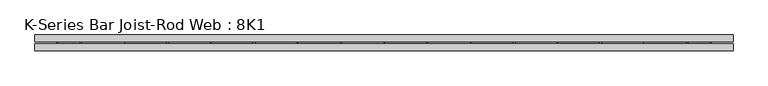
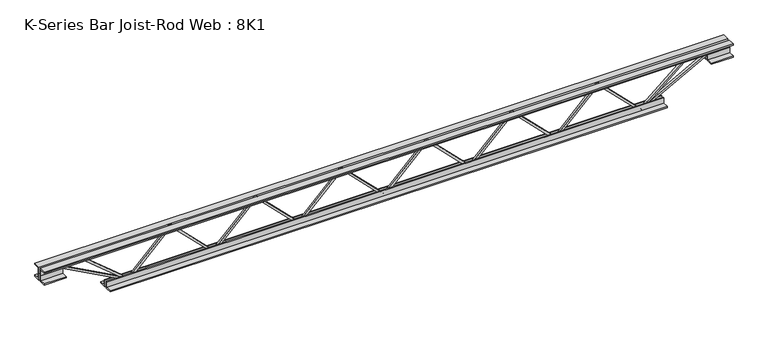
"""IFC4 building model written with IfcOpenShell, lengths in millimetres: beam geometry, K-Series Bar Joist-Rod Web : 8K1."""

import ifcopenshell
import ifcopenshell.guid

model = None  # the IFC model being written
_history = None  # IfcOwnerHistory: only IFC2X3 demands one
_inside = {}  # id of a spatial element -> (the spatial element, [elements in it])
_under = {}  # id of a project, library or spatial element -> (it, [spatial elements below it])
_declared = {}  # id of a project -> (the project, [libraries it declares])
_typed = {}  # id of a type object -> (the type object, [elements of that type])
_made_of = {}  # id of a material, layer set ... -> (it, [elements and type objects made of it])


def new_model(schema):
    """Start an empty IFC model of exactly this schema.

    Asked for "IFC4X3", IfcOpenShell would pick the latest addendum, in which some entities
    have other attributes; the version numbers below select the first issue.
    IFC2X3 requires an IfcOwnerHistory on every rooted entity: one is made here for all.
    """
    global model, _history
    if schema == "IFC4X3":
        model = ifcopenshell.file(schema_version=(4, 3, 0, 0))
    else:
        model = ifcopenshell.file(schema=schema)
    _inside.clear()
    _under.clear()
    _declared.clear()
    _typed.clear()
    _made_of.clear()
    _history = None
    if model.schema == "IFC2X3":
        org = make("IfcOrganization", Name="unknown")
        user = make(
            "IfcPersonAndOrganization",
            ThePerson=make("IfcPerson", FamilyName="unknown"),
            TheOrganization=org,
        )
        app = make(
            "IfcApplication",
            ApplicationDeveloper=org,
            Version="unknown",
            ApplicationFullName="unknown",
            ApplicationIdentifier="unknown",
        )
        _history = make(
            "IfcOwnerHistory",
            OwningUser=user,
            OwningApplication=app,
            ChangeAction="ADDED",
            CreationDate=0,
        )
    return model


def make(cls, **values):
    """One entity of the class cls with the attributes given. An attribute that is None is left unset."""
    return model.create_entity(
        cls, **{name: value for name, value in values.items() if value is not None}
    )


def rooted(cls, **values):
    """An entity with a GlobalId (a new one), such as an element, a storey or a relation."""
    return make(cls, GlobalId=ifcopenshell.guid.new(), OwnerHistory=_history, **values)


def si_unit(unit_type, name, prefix=None):
    """IfcSIUnit, for example si_unit("LENGTHUNIT", "METRE", prefix="MILLI")."""
    return make("IfcSIUnit", UnitType=unit_type, Prefix=prefix, Name=name)


def assignment(units):
    """IfcUnitAssignment: the units of a project."""
    return None if units is None else make("IfcUnitAssignment", Units=units)


def point(xyz):
    """IfcCartesianPoint."""
    return None if xyz is None else make("IfcCartesianPoint", Coordinates=xyz)


def direction(xyz):
    """IfcDirection."""
    return None if xyz is None else make("IfcDirection", DirectionRatios=xyz)


def frame(location, z_axis=None, x_axis=None):
    """IfcAxis2Placement3D, a coordinate frame: its origin and axes. An axis left out is left unset."""
    return make(
        "IfcAxis2Placement3D",
        Location=point(location),
        Axis=direction(z_axis),
        RefDirection=direction(x_axis),
    )


def origin():
    """The frame at (0, 0, 0) with its axes left unset."""
    return frame((0.0, 0.0, 0.0))


def place(relative_to, where):
    """IfcLocalPlacement: puts the frame where relative to a parent placement (None: the world)."""
    return make(
        "IfcLocalPlacement", PlacementRelTo=relative_to, RelativePlacement=where
    )


def context(
    kind, dimensions, precision=None, world=None, true_north=None, identifier=None
):
    """IfcGeometricRepresentationContext, for example the 3D "Model" context."""
    return make(
        "IfcGeometricRepresentationContext",
        ContextIdentifier=identifier,
        ContextType=kind,
        CoordinateSpaceDimension=dimensions,
        Precision=precision,
        WorldCoordinateSystem=world,
        TrueNorth=true_north,
    )


def project(units=None, contexts=None):
    """IfcProject with its units and contexts."""
    return rooted(
        "IfcProject",
        Name="project",
        RepresentationContexts=contexts,
        UnitsInContext=assignment(units),
    )


def spatial(cls, under=None, at=None, **own):
    """A site, building, storey or space (cls), placed at a placement, below another one or the project."""
    s = rooted(cls, ObjectPlacement=at, **own)
    if under is not None:
        _under.setdefault(under.id(), (under, []))[1].append(s)
    return s


def polyline(points):
    """IfcPolyline through the points."""
    return make("IfcPolyline", Points=[point(p) for p in points])


def outline(outer, holes=None, kind="AREA"):
    """IfcArbitraryClosedProfileDef: a profile drawn as a closed curve; with holes, ...WithVoids."""
    if holes is None:
        return make("IfcArbitraryClosedProfileDef", ProfileType=kind, OuterCurve=outer)
    return make(
        "IfcArbitraryProfileDefWithVoids",
        ProfileType=kind,
        OuterCurve=outer,
        InnerCurves=holes,
    )


def extrude(swept, where, along, depth):
    """IfcExtrudedAreaSolid: the profile swept, set in the frame where, extruded along a direction by depth."""
    return make(
        "IfcExtrudedAreaSolid",
        SweptArea=swept,
        Position=where,
        ExtrudedDirection=direction(along),
        Depth=depth,
    )


def shape(context_of_items, identifier, shape_type, items):
    """IfcShapeRepresentation: the items that make up one representation, for example the "Body"."""
    return make(
        "IfcShapeRepresentation",
        ContextOfItems=context_of_items,
        RepresentationIdentifier=identifier,
        RepresentationType=shape_type,
        Items=items,
    )


def source(mapping_origin, context_of_items, identifier, shape_type, items):
    """IfcRepresentationMap: a shape defined once, which mapped items show again and again."""
    return make(
        "IfcRepresentationMap",
        MappingOrigin=mapping_origin,
        MappedRepresentation=shape(context_of_items, identifier, shape_type, items),
    )


def transform(
    local_origin,
    x_axis=None,
    y_axis=None,
    z_axis=None,
    scale=None,
    scale2=None,
    scale3=None,
    uniform=True,
):
    """IfcCartesianTransformationOperator3D, or its non-uniform kind. x_axis, y_axis, z_axis: its Axis1, 2, 3."""
    if uniform:
        return make(
            "IfcCartesianTransformationOperator3D",
            Axis1=direction(x_axis),
            Axis2=direction(y_axis),
            LocalOrigin=point(local_origin),
            Scale=scale,
            Axis3=direction(z_axis),
        )
    return make(
        "IfcCartesianTransformationOperator3DnonUniform",
        Axis1=direction(x_axis),
        Axis2=direction(y_axis),
        LocalOrigin=point(local_origin),
        Scale=scale,
        Axis3=direction(z_axis),
        Scale2=scale2,
        Scale3=scale3,
    )


def mapped(mapping_source, mapping_target):
    """IfcMappedItem: shows the shape of a source again, moved by a transform."""
    return make(
        "IfcMappedItem", MappingSource=mapping_source, MappingTarget=mapping_target
    )


def made_of(thing, what):
    """Note that an element or type object is made of a material, layer set ...; save() writes the relation."""
    if what is not None:
        _made_of.setdefault(what.id(), (what, []))[1].append(thing)
    return thing


def element(
    cls,
    number,
    at=None,
    inside=None,
    cuts=None,
    type_object=None,
    material=None,
    context=None,
    identifier="Body",
    shape_type=None,
    held_by="IfcProductDefinitionShape",
    body=None,
    shapes=None,
    **own,
):
    """One element of the class cls, such as IfcWall. Its Tag is "e" and its number.

    at: its placement. inside: the storey or other place that contains it. cuts: it is an
    opening in that element (IfcRelVoidsElement). A single representation is given by context,
    identifier, shape_type and body (its items); several are given by shapes. held_by: the class
    of the entity that holds the representations. save() writes the other relations.
    """
    e = rooted(cls, Tag="e%d" % number, ObjectPlacement=at, **own)
    if body is not None:
        shapes = [shape(context, identifier, shape_type, body)]
    if shapes is not None:
        e.Representation = make(held_by, Representations=shapes)
    if inside is not None:
        _inside.setdefault(inside.id(), (inside, []))[1].append(e)
    if cuts is not None:
        rooted(
            "IfcRelVoidsElement", RelatingBuildingElement=cuts, RelatedOpeningElement=e
        )
    if type_object is not None:
        _typed.setdefault(type_object.id(), (type_object, []))[1].append(e)
    return made_of(e, material)


def aggregate(whole, parts):
    """IfcRelAggregates: a whole, such as a stair, and the parts it consists of."""
    return rooted("IfcRelAggregates", RelatingObject=whole, RelatedObjects=parts)


def save(model, path):
    """Write the relations noted so far, then the file.

    IfcRelAggregates (storeys below a building ...), IfcRelContainedInSpatialStructure (elements
    in a storey), IfcRelDefinesByType, IfcRelAssociatesMaterial and IfcRelDeclares: one each for
    every whole, place, type object, material and project.
    """
    for whole, parts in _under.values():
        aggregate(whole, parts)
    for where, things in _inside.values():
        rooted(
            "IfcRelContainedInSpatialStructure",
            RelatedElements=things,
            RelatingStructure=where,
        )
    for kind, things in _typed.values():
        rooted("IfcRelDefinesByType", RelatedObjects=things, RelatingType=kind)
    for what, things in _made_of.values():
        rooted("IfcRelAssociatesMaterial", RelatedObjects=things, RelatingMaterial=what)
    for by, libraries in _declared.values():
        rooted("IfcRelDeclares", RelatingContext=by, RelatedDefinitions=libraries)
    model.write(path)


def k_series_bar_joist_rod_web_8k1_291a3e72(model_context):
    return source(origin(), model_context, "Body", "SweptSolid", [
        extrude(outline(polyline([(-90.4875, 394.3021306), (-100.0125, 394.3021306), (-100.0125, 399.4476203), (90.4875, 590.2486857), (90.4875, 592.6577063), (-100.0125, 783.4587716), (-100.0125, 788.6042613), (-90.4875, 788.6042613), (-90.4875, 787.399751), (100.0125, 596.5986857), (100.0125, 586.3077063), (-90.4875, 395.506641), (-90.4875, 394.3021306)])), frame((0.0, -4.7625, 0.0), z_axis=(0.0, 1.0, 0.0), x_axis=(0.0, 0.0, 1.0)), (0.0, 0.0, 1.0), 9.525),
        extrude(outline(polyline([(-90.4875, 0.0), (-100.0125, 0.0), (-100.0125, 5.1454897), (90.4875, 195.946555), (90.4875, 198.3555756), (-100.0125, 389.156641), (-100.0125, 394.3021306), (-90.4875, 394.3021306), (-90.4875, 393.0976203), (100.0125, 202.296555), (100.0125, 192.0055756), (-90.4875, 1.2045103), (-90.4875, 0.0)])), frame((0.0, -4.7625, 0.0), z_axis=(0.0, 1.0, 0.0), x_axis=(0.0, 0.0, 1.0)), (0.0, 0.0, 1.0), 9.525),
        extrude(outline(polyline([(-90.4875, -394.3021306), (-100.0125, -394.3021306), (-100.0125, -389.156641), (90.4875, -198.3555756), (90.4875, -195.946555), (-100.0125, -5.1454897), (-100.0125, 0.0), (-90.4875, 0.0), (-90.4875, -1.2045103), (100.0125, -192.0055756), (100.0125, -202.296555), (-90.4875, -393.0976203), (-90.4875, -394.3021306)])), frame((0.0, -4.7625, 0.0), z_axis=(0.0, 1.0, 0.0), x_axis=(0.0, 0.0, 1.0)), (0.0, 0.0, 1.0), 9.525),
        extrude(outline(polyline([(-90.4875, -788.6042613), (-100.0125, -788.6042613), (-100.0125, -783.4587716), (90.4875, -592.6577063), (90.4875, -590.2486857), (-100.0125, -399.4476203), (-100.0125, -394.3021306), (-90.4875, -394.3021306), (-90.4875, -395.506641), (100.0125, -586.3077063), (100.0125, -596.5986857), (-90.4875, -787.399751), (-90.4875, -788.6042613)])), frame((0.0, -4.7625, 0.0), z_axis=(0.0, 1.0, 0.0), x_axis=(0.0, 0.0, 1.0)), (0.0, 0.0, 1.0), 9.525),
        extrude(outline(polyline([(-90.4875, 788.6042613), (-100.0125, 788.6042613), (-100.0125, 793.749751), (90.4875, 984.5508163), (90.4875, 986.9598369), (-100.0125, 1177.7609023), (-100.0125, 1182.9063919), (-90.4875, 1182.9063919), (-90.4875, 1181.7018816), (100.0125, 990.9008163), (100.0125, 980.6098369), (-90.4875, 789.8087716), (-90.4875, 788.6042613)])), frame((0.0, -4.7625, 0.0), z_axis=(0.0, 1.0, 0.0), x_axis=(0.0, 0.0, 1.0)), (0.0, 0.0, 1.0), 9.525),
        extrude(outline(polyline([(-90.4875, -1182.9063919), (-100.0125, -1182.9063919), (-100.0125, -1177.7609023), (90.4875, -986.9598369), (90.4875, -984.5508163), (-100.0125, -793.749751), (-100.0125, -788.6042613), (-90.4875, -788.6042613), (-90.4875, -789.8087716), (100.0125, -980.6098369), (100.0125, -990.9008163), (-90.4875, -1181.7018816), (-90.4875, -1182.9063919)])), frame((0.0, -4.7625, 0.0), z_axis=(0.0, 1.0, 0.0), x_axis=(0.0, 0.0, 1.0)), (0.0, 0.0, 1.0), 9.525),
        extrude(outline(polyline([(4.7625, 101.6), (36.5125, 101.6), (36.5125, 95.25), (11.1125, 95.25), (11.1125, 69.85), (4.7625, 69.85), (4.7625, 101.6)])), frame((-1589.3063919, 0.0, 0.0), z_axis=(1.0, 0.0, 0.0), x_axis=(0.0, 1.0, 0.0)), (0.0, 0.0, 1.0), 3178.6127839),
        extrude(outline(polyline([(-4.7625, 101.6), (-4.7625, 69.85), (-11.1125, 69.85), (-11.1125, 95.25), (-36.5125, 95.25), (-36.5125, 101.6), (-4.7625, 101.6)])), frame((-1589.3063919, 0.0, 0.0), z_axis=(1.0, 0.0, 0.0), x_axis=(0.0, 1.0, 0.0)), (0.0, 0.0, 1.0), 3178.6127839),
        extrude(outline(polyline([(-4.7625, 38.1), (-36.5125, 38.1), (-36.5125, 44.45), (-11.1125, 44.45), (-11.1125, 69.85), (-4.7625, 69.85), (-4.7625, 38.1)])), frame((-1589.3063919, 0.0, 0.0), z_axis=(1.0, 0.0, 0.0), x_axis=(0.0, 1.0, 0.0)), (0.0, 0.0, 1.0), 101.6),
        extrude(outline(polyline([(36.5125, 38.1), (4.7625, 38.1), (4.7625, 69.85), (11.1125, 69.85), (11.1125, 44.45), (36.5125, 44.45), (36.5125, 38.1)])), frame((-1589.3063919, 0.0, 0.0), z_axis=(1.0, 0.0, 0.0), x_axis=(0.0, 1.0, 0.0)), (0.0, 0.0, 1.0), 101.6),
        extrude(outline(polyline([(4.7625, 38.1), (4.7625, 69.85), (11.1125, 69.85), (11.1125, 44.45), (36.5125, 44.45), (36.5125, 38.1), (4.7625, 38.1)])), frame((1487.7063919, 0.0, 0.0), z_axis=(1.0, 0.0, 0.0), x_axis=(0.0, 1.0, 0.0)), (0.0, 0.0, 1.0), 101.6),
        extrude(outline(polyline([(-4.7625, 38.1), (-36.5125, 38.1), (-36.5125, 44.45), (-11.1125, 44.45), (-11.1125, 69.85), (-4.7625, 69.85), (-4.7625, 38.1)])), frame((1487.7063919, 0.0, 0.0), z_axis=(1.0, 0.0, 0.0), x_axis=(0.0, 1.0, 0.0)), (0.0, 0.0, 1.0), 101.6),
        extrude(outline(polyline([(4.7625, -101.6), (4.7625, -69.85), (11.1125, -69.85), (11.1125, -95.25), (36.5125, -95.25), (36.5125, -101.6), (4.7625, -101.6)])), frame((-1284.5063919, 0.0, 0.0), z_axis=(1.0, 0.0, 0.0), x_axis=(0.0, 1.0, 0.0)), (0.0, 0.0, 1.0), 2569.0127839),
        extrude(outline(polyline([(-4.7625, -101.6), (-36.5125, -101.6), (-36.5125, -95.25), (-11.1125, -95.25), (-11.1125, -69.85), (-4.7625, -69.85), (-4.7625, -101.6)])), frame((-1284.5063919, 0.0, 0.0), z_axis=(1.0, 0.0, 0.0), x_axis=(0.0, 1.0, 0.0)), (0.0, 0.0, 1.0), 2569.0127839),
        extrude(outline(polyline([(0.0, -9.525), (0.0, 0.0), (346.6425392, 0.0), (346.6425392, -9.525), (0.0, -9.525)])), frame((-1489.9746904, 4.7625, 65.662372), z_axis=(0.47628314854008014, 0.0, 0.8792919665371384), x_axis=(0.8792919665371384, 0.0, -0.47628314854008014)), (0.0, 0.0, 1.0), 9.525),
        extrude(outline(polyline([(0.0, -9.525), (0.0, 0.0), (257.1508363, 0.0), (257.1508363, -9.525), (0.0, -9.525)])), frame((-1383.115152, 4.7625, 66.1987113), z_axis=(0.6420356334036287, 0.0, 0.7666747977076078), x_axis=(0.7666747977076078, 0.0, -0.6420356334036287)), (0.0, 0.0, 1.0), 9.525),
        extrude(outline(polyline([(0.0, -9.525), (0.0, 0.0), (346.6425392, 0.0), (346.6425392, -9.525), (0.0, -9.525)])), frame((1489.9746904, -4.7625, 65.662372), z_axis=(-0.4762831485400427, 0.0, 0.8792919665371586), x_axis=(-0.8792919665371586, 0.0, -0.4762831485400427)), (0.0, 0.0, 1.0), 9.525),
        extrude(outline(polyline([(0.0, -9.525), (0.0, 0.0), (257.1508363, 0.0), (257.1508363, -9.525), (0.0, -9.525)])), frame((1383.115152, -4.7625, 66.1987113), z_axis=(-0.6420356334036003, 0.0, 0.7666747977076316), x_axis=(-0.7666747977076316, 0.0, -0.6420356334036003)), (0.0, 0.0, 1.0), 9.525),
    ])


if __name__ == "__main__":
    model = new_model("IFC4")
    model_context = context("Model", 3, world=origin())
    ifc_project = project(units=[si_unit("LENGTHUNIT", "METRE", prefix="MILLI")], contexts=[model_context])
    site = spatial("IfcSite", under=ifc_project)
    building = spatial("IfcBuilding", under=site)
    placement = place(None, origin())
    k_series_bar_joist_rod_web_8k1_shape = k_series_bar_joist_rod_web_8k1_291a3e72(model_context)
    element("IfcBeam", 1, ObjectType="K-Series Bar Joist-Rod Web : 8K1", at=placement, inside=building, context=model_context, shape_type="MappedRepresentation", body=[
        mapped(k_series_bar_joist_rod_web_8k1_shape, transform((0.0, 0.0, 0.0), x_axis=(1.0, 0.0, 0.0), y_axis=(0.0, 1.0, 0.0), z_axis=(0.0, 0.0, 1.0))),
    ])
    save(model, "model.ifc")

# Revit data of these elements
# Type "K-Series Bar Joist-Rod Web : 8K1"
#   Assembly Code = "B1010350"
#   Wt = 5.1
#   Web Thickness = 0' - 0 3/8"
#   Start Offset [instance default] = 0' - 0"
#   Start Extension [instance default] = 0' - 0"
#   Seat Length = 0' - 4"
#   Seat Depth = 0' - 2 1/2"
#   PanelArrayLength [instance default] = 21' - 4"
#   Panel [instance default] = 1' - 4"
#   End Offset [instance default] = 0' - 0"
#   End Extension [instance default] = 0' - 0"
#   End Panel = 1' - 4"
#   Cord Leg = 0' - 1 1/4"
#   Chord Thickness = 0' - 0 1/4"
#   Length [instance default] = 24' - 0"
#   Depth = 0' - 8"
#   PanelArrayNum [instance default] = 16
#   Rendering Material = none
# Element 1 (IfcBeam, "K-Series Bar Joist-Rod Web : 8K1")
#   PanelArrayLength = 7' - 9.14224"
#   Panel = 1' - 3.52371"
#   PanelArrayNum = 6
